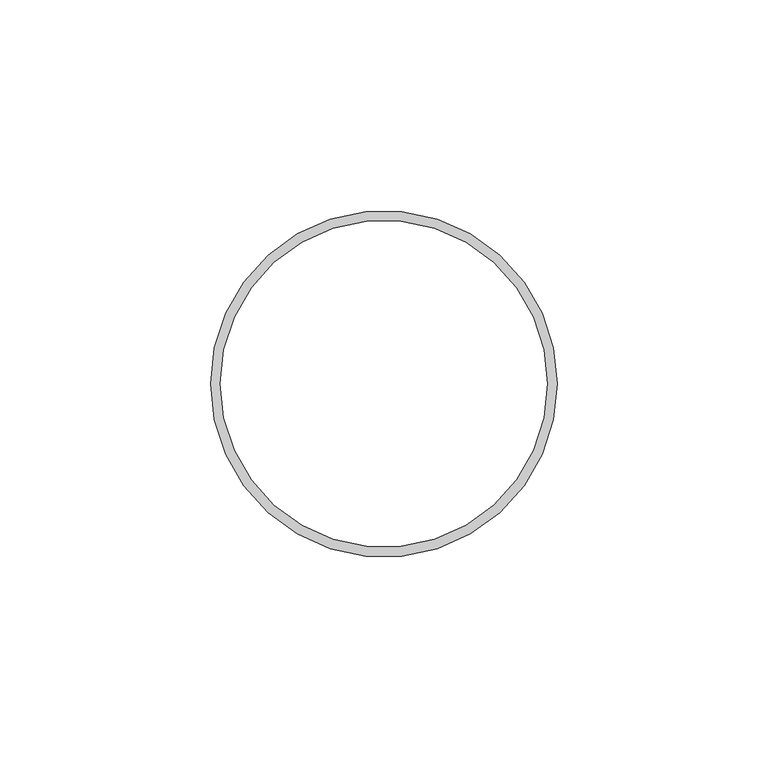
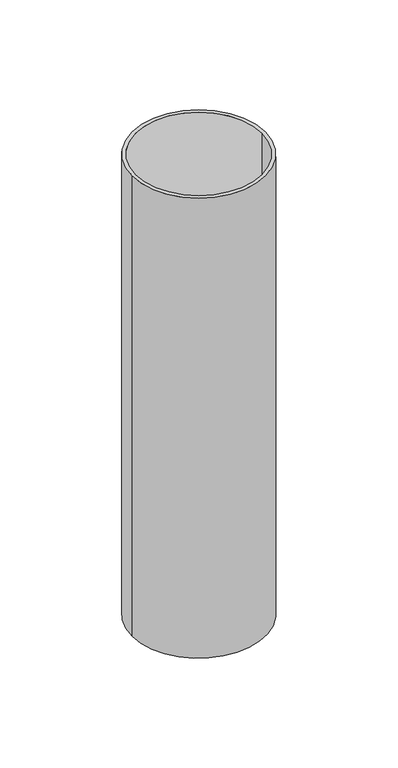
"""IFC4 building model written with IfcOpenShell, lengths in millimetres: proxy geometry, TN_ПВС 125-82_Водосточная труба : TN_ПВС 125-82_Водосточная труба."""

from ifc_helpers import new_model, si_unit, point, origin, origin_with_axes, origin_2d, place, context, project, spatial, circle_curve, trimmed, segment, composite_curve, outline, extrude, source, transform, mapped, element, save


def generic_models_4957fc4e(model_context):
    return source(origin(), model_context, "Body", "SweptSolid", [
        extrude(outline(composite_curve([segment(trimmed(circle_curve(origin_2d(), 41.1), [point((-41.1, 0.0))], [point((41.1, 0.0))], False, "CARTESIAN"), True, "CONTINUOUS"), segment(trimmed(circle_curve(origin_2d(), 41.1), [point((41.1, 0.0))], [point((-41.1, 0.0))], False, "CARTESIAN"), True, "CONTINUOUS")], self_intersect=False), holes=[composite_curve([segment(trimmed(circle_curve(origin_2d(), 38.8), [point((-38.8, 0.0))], [point((38.8, 0.0))], True, "CARTESIAN"), True, "CONTINUOUS"), segment(trimmed(circle_curve(origin_2d(), 38.8), [point((38.8, 0.0))], [point((-38.8, 0.0))], True, "CARTESIAN"), True, "CONTINUOUS")], self_intersect=False)]), origin_with_axes(), (0.0, 0.0, 1.0), 300.0),
    ])


if __name__ == "__main__":
    model = new_model("IFC4")
    model_context = context("Model", 3, world=origin())
    ifc_project = project(units=[si_unit("LENGTHUNIT", "METRE", prefix="MILLI")], contexts=[model_context])
    site = spatial("IfcSite", under=ifc_project)
    building = spatial("IfcBuilding", under=site)
    placement = place(None, origin())
    generic_models_shape = generic_models_4957fc4e(model_context)
    element("IfcBuildingElementProxy", 1, Name="TN_ПВС 125-82_Водосточная труба : TN_ПВС 125-82_Водосточная труба", ObjectType="TN_ПВС 125-82_Водосточная труба : TN_ПВС 125-82_Водосточная труба", at=placement, inside=building, context=model_context, shape_type="MappedRepresentation", body=[
        mapped(generic_models_shape, transform((0.0, 0.0, 0.0), x_axis=(1.0, 0.0, 0.0), y_axis=(0.0, 1.0, 0.0), z_axis=(0.0, 0.0, 1.0))),
    ])
    save(model, "model.ifc")

# Revit data of these elements
# Type "TN_ПВС 125-82_Водосточная труба : TN_ПВС 125-82_Водосточная труба"
#   Description = "Организует вертикальный сток дождевой воды"
#   Manufacturer = "ТехноНИКОЛЬ"
#   Model = "Комплектующие к водосточным системам"
#   URL = "https://tn-vodostok.ru/catalog/pvh/"
#   ADSK_Обозначение = "ТехноНИКОЛЬ"
#   ADSK_Наименование краткое = "Труба"
#   ADSK_Наименование = "Водосточная труба"
#   ADSK_Масса_Текст = ""
#   ADSK_Марка = ""
#   ADSK_Код изделия = ""
#   ADSK_Завод-изготовитель = "ТехноНИКОЛЬ"
#   ADSK_Единица измерения = "п.м."
#   ADSK_Группирование = "Комплектующие к водосточным системам"
#   ADSK_URL страницы изделия = "https://tn-vodostok.ru/catalog/pvh/"
#   ADSK_URL документации изделия = "https://tn-vodostok.ru/upload/iblock/c42/c427963cb77eb5c3c51f0cfb870e9e52.pdf"
#   ADSK_Размер_Диаметр = 82.2 mm
#   ADSK_Размер_Высота [instance default] = 500 mm
#   ADSK_Количество [instance default] = 0.5
#   ADSK_Материал [instance default] = TN_Пластик_Коричневый_RAL8019
#   Default Elevation = 0
# Element 1 (IfcBuildingElementProxy, "TN_ПВС 125-82_Водосточная труба : TN_ПВС 125-82_Водосточная труба")
#   ADSK_Размер_Высота = 300 mm
#   ADSK_Количество = 0.3
#   Materials on its faces: "TN_Пластик_Коричневый_RAL8019"
# Materials
#   "TN_Пластик_Коричневый_RAL8019": class "Типовые", colour RGB 61 54 53, transparency 0, Cost = 0
